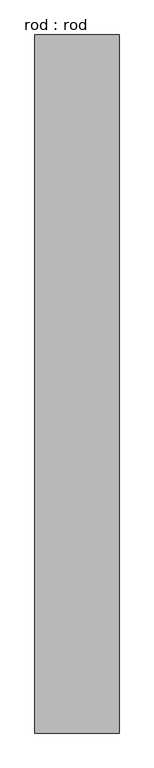
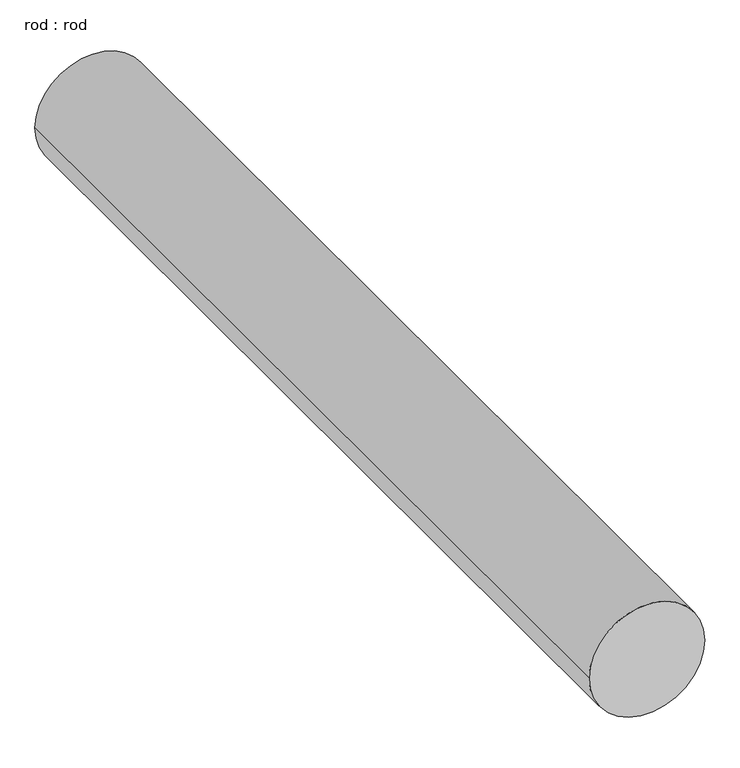
"""IFC4 building model written with IfcOpenShell, lengths in millimetres: proxy geometry, rod : rod."""

import ifcopenshell
import ifcopenshell.guid

model = None  # the IFC model being written
_history = None  # IfcOwnerHistory: only IFC2X3 demands one
_inside = {}  # id of a spatial element -> (the spatial element, [elements in it])
_under = {}  # id of a project, library or spatial element -> (it, [spatial elements below it])
_declared = {}  # id of a project -> (the project, [libraries it declares])
_typed = {}  # id of a type object -> (the type object, [elements of that type])
_made_of = {}  # id of a material, layer set ... -> (it, [elements and type objects made of it])


def new_model(schema):
    """Start an empty IFC model of exactly this schema.

    Asked for "IFC4X3", IfcOpenShell would pick the latest addendum, in which some entities
    have other attributes; the version numbers below select the first issue.
    IFC2X3 requires an IfcOwnerHistory on every rooted entity: one is made here for all.
    """
    global model, _history
    if schema == "IFC4X3":
        model = ifcopenshell.file(schema_version=(4, 3, 0, 0))
    else:
        model = ifcopenshell.file(schema=schema)
    _inside.clear()
    _under.clear()
    _declared.clear()
    _typed.clear()
    _made_of.clear()
    _history = None
    if model.schema == "IFC2X3":
        org = make("IfcOrganization", Name="unknown")
        user = make(
            "IfcPersonAndOrganization",
            ThePerson=make("IfcPerson", FamilyName="unknown"),
            TheOrganization=org,
        )
        app = make(
            "IfcApplication",
            ApplicationDeveloper=org,
            Version="unknown",
            ApplicationFullName="unknown",
            ApplicationIdentifier="unknown",
        )
        _history = make(
            "IfcOwnerHistory",
            OwningUser=user,
            OwningApplication=app,
            ChangeAction="ADDED",
            CreationDate=0,
        )
    return model


def make(cls, **values):
    """One entity of the class cls with the attributes given. An attribute that is None is left unset."""
    return model.create_entity(
        cls, **{name: value for name, value in values.items() if value is not None}
    )


def rooted(cls, **values):
    """An entity with a GlobalId (a new one), such as an element, a storey or a relation."""
    return make(cls, GlobalId=ifcopenshell.guid.new(), OwnerHistory=_history, **values)


def si_unit(unit_type, name, prefix=None):
    """IfcSIUnit, for example si_unit("LENGTHUNIT", "METRE", prefix="MILLI")."""
    return make("IfcSIUnit", UnitType=unit_type, Prefix=prefix, Name=name)


def assignment(units):
    """IfcUnitAssignment: the units of a project."""
    return None if units is None else make("IfcUnitAssignment", Units=units)


def point(xyz):
    """IfcCartesianPoint."""
    return None if xyz is None else make("IfcCartesianPoint", Coordinates=xyz)


def direction(xyz):
    """IfcDirection."""
    return None if xyz is None else make("IfcDirection", DirectionRatios=xyz)


def frame(location, z_axis=None, x_axis=None):
    """IfcAxis2Placement3D, a coordinate frame: its origin and axes. An axis left out is left unset."""
    return make(
        "IfcAxis2Placement3D",
        Location=point(location),
        Axis=direction(z_axis),
        RefDirection=direction(x_axis),
    )


def frame_2d(location, x_axis=None):
    """IfcAxis2Placement2D, a coordinate frame in the plane: its origin and x axis."""
    return make(
        "IfcAxis2Placement2D", Location=point(location), RefDirection=direction(x_axis)
    )


def origin():
    """The frame at (0, 0, 0) with its axes left unset."""
    return frame((0.0, 0.0, 0.0))


def place(relative_to, where):
    """IfcLocalPlacement: puts the frame where relative to a parent placement (None: the world)."""
    return make(
        "IfcLocalPlacement", PlacementRelTo=relative_to, RelativePlacement=where
    )


def context(
    kind, dimensions, precision=None, world=None, true_north=None, identifier=None
):
    """IfcGeometricRepresentationContext, for example the 3D "Model" context."""
    return make(
        "IfcGeometricRepresentationContext",
        ContextIdentifier=identifier,
        ContextType=kind,
        CoordinateSpaceDimension=dimensions,
        Precision=precision,
        WorldCoordinateSystem=world,
        TrueNorth=true_north,
    )


def project(units=None, contexts=None):
    """IfcProject with its units and contexts."""
    return rooted(
        "IfcProject",
        Name="project",
        RepresentationContexts=contexts,
        UnitsInContext=assignment(units),
    )


def spatial(cls, under=None, at=None, **own):
    """A site, building, storey or space (cls), placed at a placement, below another one or the project."""
    s = rooted(cls, ObjectPlacement=at, **own)
    if under is not None:
        _under.setdefault(under.id(), (under, []))[1].append(s)
    return s


def circle_curve(where, radius):
    """IfcCircle in the frame where."""
    return make("IfcCircle", Position=where, Radius=radius)


def trimmed(basis, trim1, trim2, sense, master):
    """IfcTrimmedCurve: the piece of a basis curve between two trims."""
    return make(
        "IfcTrimmedCurve",
        BasisCurve=basis,
        Trim1=trim1,
        Trim2=trim2,
        SenseAgreement=sense,
        MasterRepresentation=master,
    )


def segment(curve, same_sense, transition):
    """IfcCompositeCurveSegment."""
    return make(
        "IfcCompositeCurveSegment",
        Transition=transition,
        SameSense=same_sense,
        ParentCurve=curve,
    )


def composite_curve(segments, self_intersect=None):
    """IfcCompositeCurve: segments joined end to end."""
    return make("IfcCompositeCurve", Segments=segments, SelfIntersect=self_intersect)


def outline(outer, holes=None, kind="AREA"):
    """IfcArbitraryClosedProfileDef: a profile drawn as a closed curve; with holes, ...WithVoids."""
    if holes is None:
        return make("IfcArbitraryClosedProfileDef", ProfileType=kind, OuterCurve=outer)
    return make(
        "IfcArbitraryProfileDefWithVoids",
        ProfileType=kind,
        OuterCurve=outer,
        InnerCurves=holes,
    )


def extrude(swept, where, along, depth):
    """IfcExtrudedAreaSolid: the profile swept, set in the frame where, extruded along a direction by depth."""
    return make(
        "IfcExtrudedAreaSolid",
        SweptArea=swept,
        Position=where,
        ExtrudedDirection=direction(along),
        Depth=depth,
    )


def shape(context_of_items, identifier, shape_type, items):
    """IfcShapeRepresentation: the items that make up one representation, for example the "Body"."""
    return make(
        "IfcShapeRepresentation",
        ContextOfItems=context_of_items,
        RepresentationIdentifier=identifier,
        RepresentationType=shape_type,
        Items=items,
    )


def source(mapping_origin, context_of_items, identifier, shape_type, items):
    """IfcRepresentationMap: a shape defined once, which mapped items show again and again."""
    return make(
        "IfcRepresentationMap",
        MappingOrigin=mapping_origin,
        MappedRepresentation=shape(context_of_items, identifier, shape_type, items),
    )


def transform(
    local_origin,
    x_axis=None,
    y_axis=None,
    z_axis=None,
    scale=None,
    scale2=None,
    scale3=None,
    uniform=True,
):
    """IfcCartesianTransformationOperator3D, or its non-uniform kind. x_axis, y_axis, z_axis: its Axis1, 2, 3."""
    if uniform:
        return make(
            "IfcCartesianTransformationOperator3D",
            Axis1=direction(x_axis),
            Axis2=direction(y_axis),
            LocalOrigin=point(local_origin),
            Scale=scale,
            Axis3=direction(z_axis),
        )
    return make(
        "IfcCartesianTransformationOperator3DnonUniform",
        Axis1=direction(x_axis),
        Axis2=direction(y_axis),
        LocalOrigin=point(local_origin),
        Scale=scale,
        Axis3=direction(z_axis),
        Scale2=scale2,
        Scale3=scale3,
    )


def mapped(mapping_source, mapping_target):
    """IfcMappedItem: shows the shape of a source again, moved by a transform."""
    return make(
        "IfcMappedItem", MappingSource=mapping_source, MappingTarget=mapping_target
    )


def made_of(thing, what):
    """Note that an element or type object is made of a material, layer set ...; save() writes the relation."""
    if what is not None:
        _made_of.setdefault(what.id(), (what, []))[1].append(thing)
    return thing


def element(
    cls,
    number,
    at=None,
    inside=None,
    cuts=None,
    type_object=None,
    material=None,
    context=None,
    identifier="Body",
    shape_type=None,
    held_by="IfcProductDefinitionShape",
    body=None,
    shapes=None,
    **own,
):
    """One element of the class cls, such as IfcWall. Its Tag is "e" and its number.

    at: its placement. inside: the storey or other place that contains it. cuts: it is an
    opening in that element (IfcRelVoidsElement). A single representation is given by context,
    identifier, shape_type and body (its items); several are given by shapes. held_by: the class
    of the entity that holds the representations. save() writes the other relations.
    """
    e = rooted(cls, Tag="e%d" % number, ObjectPlacement=at, **own)
    if body is not None:
        shapes = [shape(context, identifier, shape_type, body)]
    if shapes is not None:
        e.Representation = make(held_by, Representations=shapes)
    if inside is not None:
        _inside.setdefault(inside.id(), (inside, []))[1].append(e)
    if cuts is not None:
        rooted(
            "IfcRelVoidsElement", RelatingBuildingElement=cuts, RelatedOpeningElement=e
        )
    if type_object is not None:
        _typed.setdefault(type_object.id(), (type_object, []))[1].append(e)
    return made_of(e, material)


def aggregate(whole, parts):
    """IfcRelAggregates: a whole, such as a stair, and the parts it consists of."""
    return rooted("IfcRelAggregates", RelatingObject=whole, RelatedObjects=parts)


def save(model, path):
    """Write the relations noted so far, then the file.

    IfcRelAggregates (storeys below a building ...), IfcRelContainedInSpatialStructure (elements
    in a storey), IfcRelDefinesByType, IfcRelAssociatesMaterial and IfcRelDeclares: one each for
    every whole, place, type object, material and project.
    """
    for whole, parts in _under.values():
        aggregate(whole, parts)
    for where, things in _inside.values():
        rooted(
            "IfcRelContainedInSpatialStructure",
            RelatedElements=things,
            RelatingStructure=where,
        )
    for kind, things in _typed.values():
        rooted("IfcRelDefinesByType", RelatedObjects=things, RelatingType=kind)
    for what, things in _made_of.values():
        rooted("IfcRelAssociatesMaterial", RelatedObjects=things, RelatingMaterial=what)
    for by, libraries in _declared.values():
        rooted("IfcRelDeclares", RelatingContext=by, RelatedDefinitions=libraries)
    model.write(path)


def rod_rod_6ce27506(model_context):
    return source(origin(), model_context, "Body", "SweptSolid", [
        extrude(outline(composite_curve([segment(trimmed(circle_curve(frame_2d((0.0108462, 0.0)), 200.0), [point((0.0108462, 200.0))], [point((0.0108462, -200.0))], False, "CARTESIAN"), True, "CONTINUOUS"), segment(trimmed(circle_curve(frame_2d((0.0108462, 0.0)), 200.0), [point((0.0108462, -200.0))], [point((0.0108462, 200.0))], False, "CARTESIAN"), True, "CONTINUOUS")], self_intersect=False)), frame((0.0, 2432.7286153, 0.0), z_axis=(0.0, 1.0, 0.0), x_axis=(0.0, 0.0, 1.0)), (0.0, 0.0, 1.0), 3320.0),
    ])


if __name__ == "__main__":
    model = new_model("IFC4")
    model_context = context("Model", 3, world=origin())
    ifc_project = project(units=[si_unit("LENGTHUNIT", "METRE", prefix="MILLI")], contexts=[model_context])
    site = spatial("IfcSite", under=ifc_project)
    building = spatial("IfcBuilding", under=site)
    placement = place(None, origin())
    rod_rod_shape = rod_rod_6ce27506(model_context)
    element("IfcBuildingElementProxy", 1, Name="rod : rod", ObjectType="rod : rod", at=placement, inside=building, context=model_context, shape_type="MappedRepresentation", body=[
        mapped(rod_rod_shape, transform((0.0, 0.0, 0.0), x_axis=(1.0, 0.0, 0.0), y_axis=(0.0, 1.0, 0.0), z_axis=(0.0, 0.0, 1.0))),
    ])
    save(model, "model.ifc")

# Revit data of these elements
# Type "rod : rod"
#   Default Elevation = 0
